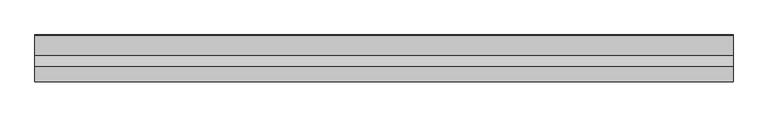
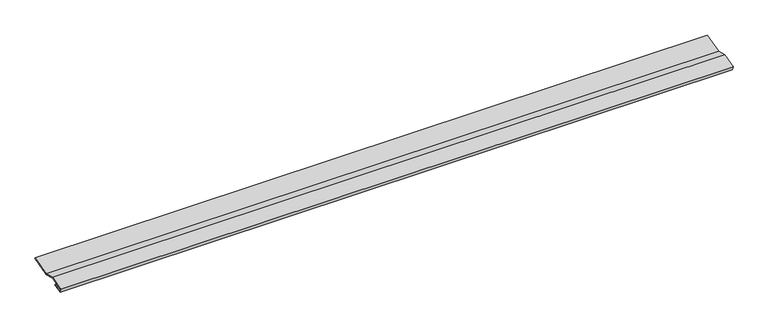
"""IFC4 building model written with IfcOpenShell, lengths in millimetres: proxy geometry, Gutter @ Roof005 : Gutter @ Roof005."""

from ifc_helpers import new_model, si_unit, frame, origin, place, context, project, spatial, polyline, outline, extrude, source, transform, mapped, element, save


def generic_models_580e674c(model_context):
    return source(origin(), model_context, "Body", "SweptSolid", [
        extrude(outline(polyline([(-5160.156595, 42852.6220122), (-5188.0399366, 42845.4152197), (-5191.2190148, 42857.6672839), (-5148.076519, 42868.8615907), (-5116.0538772, 42860.7718241), (-5057.619141, 42875.875), (-5056.9835337, 42873.4158124), (-5116.0466964, 42858.150212), (-5148.0693383, 42866.2399786), (-5188.1324915, 42855.8851642), (-5186.2186842, 42848.5094129), (-5160.7922022, 42855.0811997), (-5160.156595, 42852.6220122)])), frame((12382.7678845, 0.0, 0.0), z_axis=(1.0, 0.0, 0.0), x_axis=(0.0, 1.0, 0.0)), (0.0, 0.0, 1.0), 2000.25),
    ])


if __name__ == "__main__":
    model = new_model("IFC4")
    model_context = context("Model", 3, world=origin())
    ifc_project = project(units=[si_unit("LENGTHUNIT", "METRE", prefix="MILLI")], contexts=[model_context])
    site = spatial("IfcSite", under=ifc_project)
    building = spatial("IfcBuilding", under=site)
    placement = place(None, origin())
    generic_models_shape = generic_models_580e674c(model_context)
    element("IfcBuildingElementProxy", 1, Name="Gutter @ Roof005 : Gutter @ Roof005", ObjectType="Gutter @ Roof005 : Gutter @ Roof005", at=placement, inside=building, context=model_context, shape_type="MappedRepresentation", body=[
        mapped(generic_models_shape, transform((0.0, 0.0, 0.0), x_axis=(1.0, 0.0, 0.0), y_axis=(0.0, 1.0, 0.0), z_axis=(0.0, 0.0, 1.0))),
    ])
    save(model, "model.ifc")

# Revit data of these elements
# Type "Gutter @ Roof005 : Gutter @ Roof005"
#   NameOverride = "Gutter @ Roof005"
# Element 1 (IfcBuildingElementProxy, "Gutter @ Roof005 : Gutter @ Roof005")
#   Materials on its faces: "CONT. SEAMLESS 16 GA COPPER BRAKE METAL GUTTER"
# Materials
#   "CONT. SEAMLESS 16 GA COPPER BRAKE METAL GUTTER": class "Unassigned", colour RGB 128 128 128, transparency 0
